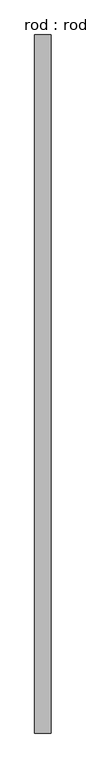
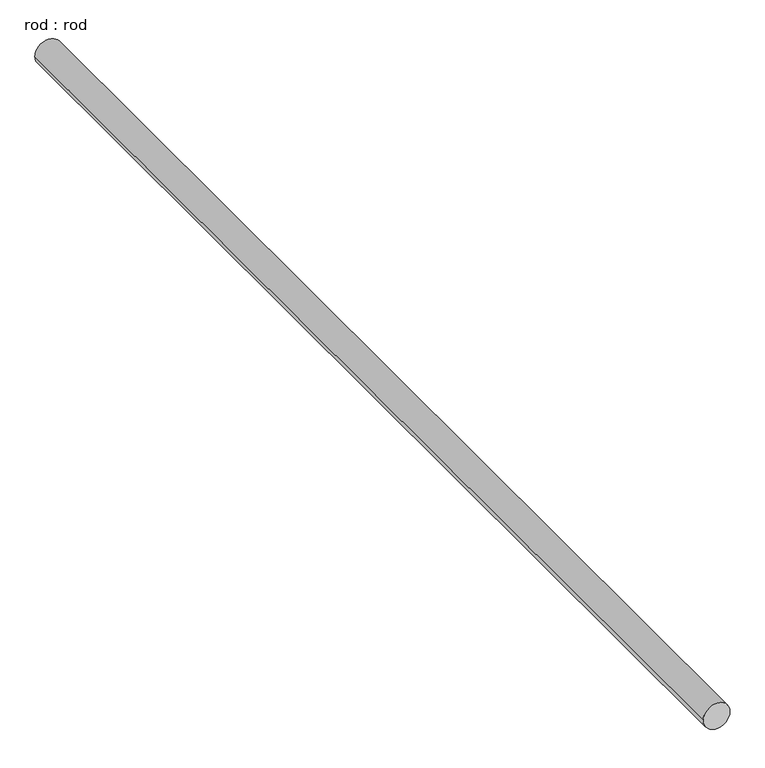
"""IFC4 building model written with IfcOpenShell, lengths in millimetres: proxy geometry, rod : rod."""

import ifcopenshell
import ifcopenshell.guid

model = None  # the IFC model being written
_history = None  # IfcOwnerHistory: only IFC2X3 demands one
_inside = {}  # id of a spatial element -> (the spatial element, [elements in it])
_under = {}  # id of a project, library or spatial element -> (it, [spatial elements below it])
_declared = {}  # id of a project -> (the project, [libraries it declares])
_typed = {}  # id of a type object -> (the type object, [elements of that type])
_made_of = {}  # id of a material, layer set ... -> (it, [elements and type objects made of it])


def new_model(schema):
    """Start an empty IFC model of exactly this schema.

    Asked for "IFC4X3", IfcOpenShell would pick the latest addendum, in which some entities
    have other attributes; the version numbers below select the first issue.
    IFC2X3 requires an IfcOwnerHistory on every rooted entity: one is made here for all.
    """
    global model, _history
    if schema == "IFC4X3":
        model = ifcopenshell.file(schema_version=(4, 3, 0, 0))
    else:
        model = ifcopenshell.file(schema=schema)
    _inside.clear()
    _under.clear()
    _declared.clear()
    _typed.clear()
    _made_of.clear()
    _history = None
    if model.schema == "IFC2X3":
        org = make("IfcOrganization", Name="unknown")
        user = make(
            "IfcPersonAndOrganization",
            ThePerson=make("IfcPerson", FamilyName="unknown"),
            TheOrganization=org,
        )
        app = make(
            "IfcApplication",
            ApplicationDeveloper=org,
            Version="unknown",
            ApplicationFullName="unknown",
            ApplicationIdentifier="unknown",
        )
        _history = make(
            "IfcOwnerHistory",
            OwningUser=user,
            OwningApplication=app,
            ChangeAction="ADDED",
            CreationDate=0,
        )
    return model


def make(cls, **values):
    """One entity of the class cls with the attributes given. An attribute that is None is left unset."""
    return model.create_entity(
        cls, **{name: value for name, value in values.items() if value is not None}
    )


def rooted(cls, **values):
    """An entity with a GlobalId (a new one), such as an element, a storey or a relation."""
    return make(cls, GlobalId=ifcopenshell.guid.new(), OwnerHistory=_history, **values)


def si_unit(unit_type, name, prefix=None):
    """IfcSIUnit, for example si_unit("LENGTHUNIT", "METRE", prefix="MILLI")."""
    return make("IfcSIUnit", UnitType=unit_type, Prefix=prefix, Name=name)


def assignment(units):
    """IfcUnitAssignment: the units of a project."""
    return None if units is None else make("IfcUnitAssignment", Units=units)


def point(xyz):
    """IfcCartesianPoint."""
    return None if xyz is None else make("IfcCartesianPoint", Coordinates=xyz)


def direction(xyz):
    """IfcDirection."""
    return None if xyz is None else make("IfcDirection", DirectionRatios=xyz)


def frame(location, z_axis=None, x_axis=None):
    """IfcAxis2Placement3D, a coordinate frame: its origin and axes. An axis left out is left unset."""
    return make(
        "IfcAxis2Placement3D",
        Location=point(location),
        Axis=direction(z_axis),
        RefDirection=direction(x_axis),
    )


def frame_2d(location, x_axis=None):
    """IfcAxis2Placement2D, a coordinate frame in the plane: its origin and x axis."""
    return make(
        "IfcAxis2Placement2D", Location=point(location), RefDirection=direction(x_axis)
    )


def origin():
    """The frame at (0, 0, 0) with its axes left unset."""
    return frame((0.0, 0.0, 0.0))


def place(relative_to, where):
    """IfcLocalPlacement: puts the frame where relative to a parent placement (None: the world)."""
    return make(
        "IfcLocalPlacement", PlacementRelTo=relative_to, RelativePlacement=where
    )


def context(
    kind, dimensions, precision=None, world=None, true_north=None, identifier=None
):
    """IfcGeometricRepresentationContext, for example the 3D "Model" context."""
    return make(
        "IfcGeometricRepresentationContext",
        ContextIdentifier=identifier,
        ContextType=kind,
        CoordinateSpaceDimension=dimensions,
        Precision=precision,
        WorldCoordinateSystem=world,
        TrueNorth=true_north,
    )


def project(units=None, contexts=None):
    """IfcProject with its units and contexts."""
    return rooted(
        "IfcProject",
        Name="project",
        RepresentationContexts=contexts,
        UnitsInContext=assignment(units),
    )


def spatial(cls, under=None, at=None, **own):
    """A site, building, storey or space (cls), placed at a placement, below another one or the project."""
    s = rooted(cls, ObjectPlacement=at, **own)
    if under is not None:
        _under.setdefault(under.id(), (under, []))[1].append(s)
    return s


def circle_curve(where, radius):
    """IfcCircle in the frame where."""
    return make("IfcCircle", Position=where, Radius=radius)


def trimmed(basis, trim1, trim2, sense, master):
    """IfcTrimmedCurve: the piece of a basis curve between two trims."""
    return make(
        "IfcTrimmedCurve",
        BasisCurve=basis,
        Trim1=trim1,
        Trim2=trim2,
        SenseAgreement=sense,
        MasterRepresentation=master,
    )


def segment(curve, same_sense, transition):
    """IfcCompositeCurveSegment."""
    return make(
        "IfcCompositeCurveSegment",
        Transition=transition,
        SameSense=same_sense,
        ParentCurve=curve,
    )


def composite_curve(segments, self_intersect=None):
    """IfcCompositeCurve: segments joined end to end."""
    return make("IfcCompositeCurve", Segments=segments, SelfIntersect=self_intersect)


def outline(outer, holes=None, kind="AREA"):
    """IfcArbitraryClosedProfileDef: a profile drawn as a closed curve; with holes, ...WithVoids."""
    if holes is None:
        return make("IfcArbitraryClosedProfileDef", ProfileType=kind, OuterCurve=outer)
    return make(
        "IfcArbitraryProfileDefWithVoids",
        ProfileType=kind,
        OuterCurve=outer,
        InnerCurves=holes,
    )


def extrude(swept, where, along, depth):
    """IfcExtrudedAreaSolid: the profile swept, set in the frame where, extruded along a direction by depth."""
    return make(
        "IfcExtrudedAreaSolid",
        SweptArea=swept,
        Position=where,
        ExtrudedDirection=direction(along),
        Depth=depth,
    )


def shape(context_of_items, identifier, shape_type, items):
    """IfcShapeRepresentation: the items that make up one representation, for example the "Body"."""
    return make(
        "IfcShapeRepresentation",
        ContextOfItems=context_of_items,
        RepresentationIdentifier=identifier,
        RepresentationType=shape_type,
        Items=items,
    )


def source(mapping_origin, context_of_items, identifier, shape_type, items):
    """IfcRepresentationMap: a shape defined once, which mapped items show again and again."""
    return make(
        "IfcRepresentationMap",
        MappingOrigin=mapping_origin,
        MappedRepresentation=shape(context_of_items, identifier, shape_type, items),
    )


def transform(
    local_origin,
    x_axis=None,
    y_axis=None,
    z_axis=None,
    scale=None,
    scale2=None,
    scale3=None,
    uniform=True,
):
    """IfcCartesianTransformationOperator3D, or its non-uniform kind. x_axis, y_axis, z_axis: its Axis1, 2, 3."""
    if uniform:
        return make(
            "IfcCartesianTransformationOperator3D",
            Axis1=direction(x_axis),
            Axis2=direction(y_axis),
            LocalOrigin=point(local_origin),
            Scale=scale,
            Axis3=direction(z_axis),
        )
    return make(
        "IfcCartesianTransformationOperator3DnonUniform",
        Axis1=direction(x_axis),
        Axis2=direction(y_axis),
        LocalOrigin=point(local_origin),
        Scale=scale,
        Axis3=direction(z_axis),
        Scale2=scale2,
        Scale3=scale3,
    )


def mapped(mapping_source, mapping_target):
    """IfcMappedItem: shows the shape of a source again, moved by a transform."""
    return make(
        "IfcMappedItem", MappingSource=mapping_source, MappingTarget=mapping_target
    )


def made_of(thing, what):
    """Note that an element or type object is made of a material, layer set ...; save() writes the relation."""
    if what is not None:
        _made_of.setdefault(what.id(), (what, []))[1].append(thing)
    return thing


def element(
    cls,
    number,
    at=None,
    inside=None,
    cuts=None,
    type_object=None,
    material=None,
    context=None,
    identifier="Body",
    shape_type=None,
    held_by="IfcProductDefinitionShape",
    body=None,
    shapes=None,
    **own,
):
    """One element of the class cls, such as IfcWall. Its Tag is "e" and its number.

    at: its placement. inside: the storey or other place that contains it. cuts: it is an
    opening in that element (IfcRelVoidsElement). A single representation is given by context,
    identifier, shape_type and body (its items); several are given by shapes. held_by: the class
    of the entity that holds the representations. save() writes the other relations.
    """
    e = rooted(cls, Tag="e%d" % number, ObjectPlacement=at, **own)
    if body is not None:
        shapes = [shape(context, identifier, shape_type, body)]
    if shapes is not None:
        e.Representation = make(held_by, Representations=shapes)
    if inside is not None:
        _inside.setdefault(inside.id(), (inside, []))[1].append(e)
    if cuts is not None:
        rooted(
            "IfcRelVoidsElement", RelatingBuildingElement=cuts, RelatedOpeningElement=e
        )
    if type_object is not None:
        _typed.setdefault(type_object.id(), (type_object, []))[1].append(e)
    return made_of(e, material)


def aggregate(whole, parts):
    """IfcRelAggregates: a whole, such as a stair, and the parts it consists of."""
    return rooted("IfcRelAggregates", RelatingObject=whole, RelatedObjects=parts)


def save(model, path):
    """Write the relations noted so far, then the file.

    IfcRelAggregates (storeys below a building ...), IfcRelContainedInSpatialStructure (elements
    in a storey), IfcRelDefinesByType, IfcRelAssociatesMaterial and IfcRelDeclares: one each for
    every whole, place, type object, material and project.
    """
    for whole, parts in _under.values():
        aggregate(whole, parts)
    for where, things in _inside.values():
        rooted(
            "IfcRelContainedInSpatialStructure",
            RelatedElements=things,
            RelatingStructure=where,
        )
    for kind, things in _typed.values():
        rooted("IfcRelDefinesByType", RelatedObjects=things, RelatingType=kind)
    for what, things in _made_of.values():
        rooted("IfcRelAssociatesMaterial", RelatedObjects=things, RelatingMaterial=what)
    for by, libraries in _declared.values():
        rooted("IfcRelDeclares", RelatingContext=by, RelatedDefinitions=libraries)
    model.write(path)


def rod_rod_d9982ffb(model_context):
    return source(origin(), model_context, "Body", "SweptSolid", [
        extrude(outline(composite_curve([segment(trimmed(circle_curve(frame_2d((0.0108462, 0.0)), 200.0), [point((0.0108462, 200.0))], [point((0.0108462, -200.0))], False, "CARTESIAN"), True, "CONTINUOUS"), segment(trimmed(circle_curve(frame_2d((0.0108462, 0.0)), 200.0), [point((0.0108462, -200.0))], [point((0.0108462, 200.0))], False, "CARTESIAN"), True, "CONTINUOUS")], self_intersect=False)), frame((0.0, -4499.1977594, 0.0), z_axis=(0.0, 1.0, 0.0), x_axis=(0.0, 0.0, 1.0)), (0.0, 0.0, 1.0), 17183.8527494),
    ])


if __name__ == "__main__":
    model = new_model("IFC4")
    model_context = context("Model", 3, world=origin())
    ifc_project = project(units=[si_unit("LENGTHUNIT", "METRE", prefix="MILLI")], contexts=[model_context])
    site = spatial("IfcSite", under=ifc_project)
    building = spatial("IfcBuilding", under=site)
    placement = place(None, origin())
    rod_rod_shape = rod_rod_d9982ffb(model_context)
    element("IfcBuildingElementProxy", 1, Name="rod : rod", ObjectType="rod : rod", at=placement, inside=building, context=model_context, shape_type="MappedRepresentation", body=[
        mapped(rod_rod_shape, transform((0.0, 0.0, 0.0), x_axis=(1.0, 0.0, 0.0), y_axis=(0.0, 1.0, 0.0), z_axis=(0.0, 0.0, 1.0))),
    ])
    save(model, "model.ifc")

# Revit data of these elements
# Type "rod : rod"
#   Default Elevation = 0
